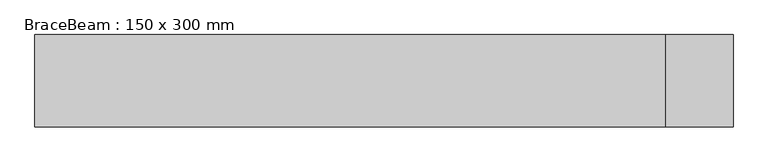
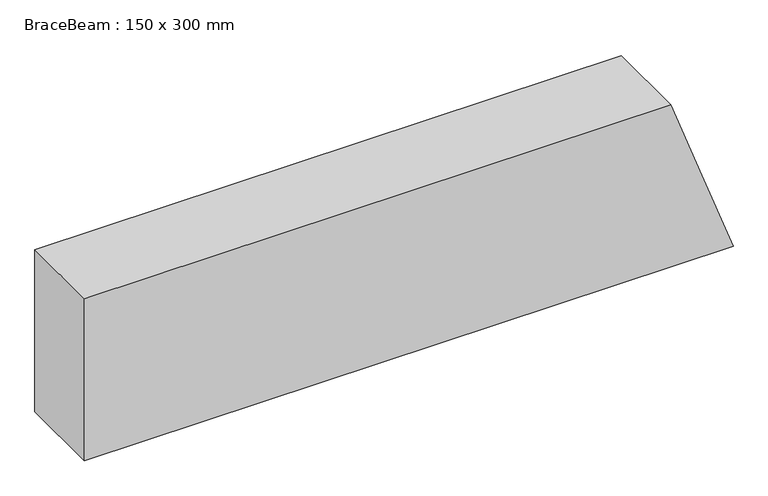
"""IFC4 building model written with IfcOpenShell, lengths in millimetres: beam geometry, BraceBeam : 150 x 300 mm."""

from ifc_helpers import new_model, si_unit, origin, place, context, project, spatial, faceted_brep, source, transform, mapped, element, save


def bracebeam_150_x_300_mm_f5e97f46(model_context):
    return source(origin(), model_context, "Body", "Brep", [
        faceted_brep([(-545.6357531, -75.0, -150.0), (-545.6357531, 75.0, -150.0), (590.6046224, 75.0, -150.0), (590.6046224, -75.0, -150.0), (-545.6357531, 75.0, 150.0), (481.4135521, 75.0, 150.0), (536.0090872, 75.0, 0.0), (-545.6357531, -75.0, 150.0), (481.4135521, -75.0, 150.0), (536.0090872, -75.0, 0.0)], [[[0, 1, 2, 3]], [[1, 4, 5, 6, 2]], [[4, 7, 8, 5]], [[7, 0, 3, 9, 8]], [[7, 4, 1, 0]], [[5, 8, 9, 3, 2, 6]]]),
    ])


if __name__ == "__main__":
    model = new_model("IFC4")
    model_context = context("Model", 3, world=origin())
    ifc_project = project(units=[si_unit("LENGTHUNIT", "METRE", prefix="MILLI")], contexts=[model_context])
    site = spatial("IfcSite", under=ifc_project)
    building = spatial("IfcBuilding", under=site)
    placement = place(None, origin())
    bracebeam_150_x_300_mm_shape = bracebeam_150_x_300_mm_f5e97f46(model_context)
    element("IfcBeam", 1, ObjectType="BraceBeam : 150 x 300 mm", at=placement, inside=building, context=model_context, shape_type="MappedRepresentation", body=[
        mapped(bracebeam_150_x_300_mm_shape, transform((0.0, 0.0, 0.0), x_axis=(1.0, 0.0, 0.0), y_axis=(0.0, 1.0, 0.0), z_axis=(0.0, 0.0, 1.0))),
    ])
    save(model, "model.ifc")

# Revit data of these elements
# Type "BraceBeam : 150 x 300 mm"
#   ExpertTruss = "Height\th\r\nWidth\tb"
#   Name [instance default] = ""
#   m [instance default] = 0 mm
#   ip_c_cut_control [instance default] = 1300 mm
#   ip_c_cut [instance default] = 1300 mm
#   h_fix [instance default] = 900 mm
#   d/2 [instance default] = 1750 mm
#   c_cut_incl [instance default] = -1000 mm
#   c_cut [instance default] = 0 mm
#   beta0_2 [instance default] = 90.00°
#   beta0_1 [instance default] = 90.00°
#   alfaMax [instance default] = 0.00°
#   alfa0_2 [instance default] = 90.00°
#   ZOffsetStr_0 [instance default] = 150 mm
#   ZOffsetStr [instance default] = 0 mm
#   ZOffsetEnd_0 [instance default] = 150 mm
#   ZOffsetEnd [instance default] = 0 mm
#   Beta2 [instance default] = 0.00°
#   Beta1 [instance default] = 0.00°
#   Alfa_str [instance default] = 0.00°
#   Alfa_cut_control [instance default] = 90.00°
#   Alfa_cut [instance default] = 90.00°
#   AlfaMAX [instance default] = 0.00°
#   Alfa2_0 [instance default] = 0.00°
#   Alfa2 [instance default] = 0.00°
#   Alfa1_0 [instance default] = 0.00°
#   Alfa1 [instance default] = 0.00°
#   A_max_Str [instance default] = 0.00°
#   h_void [instance default] = 3000 mm
#   beam_L_0 [instance default] = 100 mm
#   beam_L [instance default] = 0 mm
#   b_void [instance default] = 160 mm
#   alfa0_1 [instance default] = 90.00°
#   b = 150 mm
#   YOffsetStr [instance default] = 0 mm
#   YOffsetEnd [instance default] = 0 mm
#   XOffsetStr_0 [instance default] = 3500 mm
#   XOffsetStr [instance default] = 0 mm
#   XOffsetEnd_0 [instance default] = 3500 mm
#   XOffsetEnd [instance default] = 0 mm
#   L_void_0 [instance default] = 100 mm
#   L_void [instance default] = 0 mm
#   E2 [instance default] = 0.00°
#   E1 [instance default] = 0.00°
#   Length [instance default] = 3500 mm
#   h = 300 mm
#   Alfa [instance default] = 0.00°
#   A_max_End [instance default] = 0.00°
#   A_max [instance default] = 0.00°
#   A4 [instance default] = 0.00°
#   A3 [instance default] = 0.00°
#   A2 [instance default] = 0.00°
#   A1 [instance default] = 0.00°
#   BetaAngles [instance default] = no
#   Material [instance default] = Wood Standard
# Element 1 (IfcBeam, "BraceBeam : 150 x 300 mm")
#   d/2 = 700.438 mm
#   beta0_2 = 70.00°
#   alfaMax = -20.00°
#   alfa0_2 = 70.00°
#   AlfaMAX = -20.00°
#   Alfa2_0 = -20.00°
#   Alfa2 = -20.00°
#   h_void = 4091.911 mm
#   beam_L_0 = 873.529 mm
#   beam_L = 873.529 mm
#   XOffsetStr_0 = 1250.877 mm
#   XOffsetStr = 150 mm
#   XOffsetEnd_0 = 1241.25 mm
#   XOffsetEnd = 159.627 mm
#   L_void_0 = 2064.996 mm
#   L_void = 2064.996 mm
#   Materials on its faces: "Wood Standard"
# Materials
#   "Wood Standard": class "Drewno", colour RGB 196 146 67, transparency 0, Cost = 0
